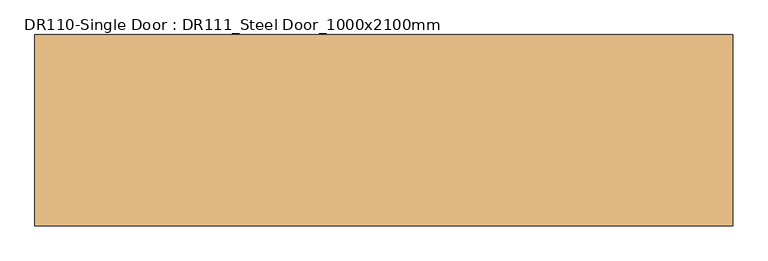
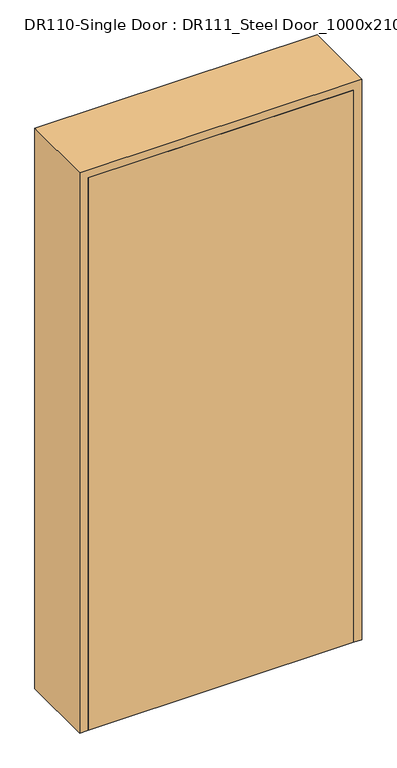
"""IFC4 building model written with IfcOpenShell, lengths in millimetres: door geometry, DR110-Single Door : DR111_Steel Door_1000x2100mm."""

from ifc_helpers import new_model, si_unit, origin, origin_with_axes, place, context, project, spatial, polyline, outline, extrude, faceted_brep, source, transform, mapped, element, save


def dr110_single_door_dr111_steel_door_1000x2100mm_c730d40a(model_context):
    return source(origin(), model_context, "Body", "SolidModel", [
        extrude(outline(polyline([(470.0, -137.0), (-470.0, -137.0), (-470.0, -102.0), (470.0, -102.0), (470.0, -137.0)])), origin_with_axes(), (0.0, 0.0, 1.0), 2070.0),
        faceted_brep([(470.0, -137.0, 0.0), (470.0, -102.0, 0.0), (450.0, -102.0, 0.0), (450.0, 102.0, 0.0), (470.0, 102.0, 0.0), (470.0, 137.0, 0.0), (500.0, 137.0, 0.0), (500.0, -137.0, 0.0), (500.0, -137.0, 2100.0), (-500.0, -137.0, 2100.0), (-500.0, -137.0, 0.0), (-470.0, -137.0, 0.0), (-470.0, -137.0, 2070.0), (470.0, -137.0, 2070.0), (500.0, 137.0, 2100.0), (470.0, 137.0, 2070.0), (-470.0, 137.0, 2070.0), (-470.0, 137.0, 0.0), (-500.0, 137.0, 0.0), (-500.0, 137.0, 2100.0), (470.0, 102.0, 2070.0), (450.0, 102.0, 2050.0), (-450.0, 102.0, 2050.0), (-450.0, 102.0, 0.0), (-470.0, 102.0, 0.0), (-470.0, 102.0, 2070.0), (450.0, -102.0, 2050.0), (470.0, -102.0, 2070.0), (-470.0, -102.0, 2070.0), (-470.0, -102.0, 0.0), (-450.0, -102.0, 0.0), (-450.0, -102.0, 2050.0)], [[[0, 1, 2, 3, 4, 5, 6, 7]], [[7, 8, 9, 10, 11, 12, 13, 0]], [[6, 14, 8, 7]], [[5, 15, 16, 17, 18, 19, 14, 6]], [[4, 20, 15, 5]], [[3, 21, 22, 23, 24, 25, 20, 4]], [[2, 26, 21, 3]], [[1, 27, 28, 29, 30, 31, 26, 2]], [[0, 13, 27, 1]], [[12, 11, 29, 28]], [[11, 10, 18, 17, 24, 23, 30, 29]], [[19, 18, 10, 9]], [[25, 24, 17, 16]], [[31, 30, 23, 22]], [[14, 19, 9, 8]], [[20, 25, 16, 15]], [[26, 31, 22, 21]], [[13, 12, 28, 27]]]),
    ])


if __name__ == "__main__":
    model = new_model("IFC4")
    model_context = context("Model", 3, world=origin())
    ifc_project = project(units=[si_unit("LENGTHUNIT", "METRE", prefix="MILLI")], contexts=[model_context])
    site = spatial("IfcSite", under=ifc_project)
    building = spatial("IfcBuilding", under=site)
    placement = place(None, origin())
    dr110_single_door_dr111_steel_door_1000x2100mm_shape = dr110_single_door_dr111_steel_door_1000x2100mm_c730d40a(model_context)
    element("IfcDoor", 1, ObjectType="DR110-Single Door : DR111_Steel Door_1000x2100mm", at=placement, inside=building, context=model_context, shape_type="MappedRepresentation", body=[
        mapped(dr110_single_door_dr111_steel_door_1000x2100mm_shape, transform((0.0, 0.0, 0.0), x_axis=(1.0, 0.0, 0.0), y_axis=(0.0, 1.0, 0.0), z_axis=(0.0, 0.0, 1.0))),
    ])
    save(model, "model.ifc")

# Revit data of these elements
# Type "DR110-Single Door : DR111_Steel Door_1000x2100mm"
#   Type Mark = "SD"
#   Analytic Construction = "<None>"
#   프레임 투영 외부. = 25 mm
#   프레임 투영 내부. = 25 mm
#   프레임 폭 = 75 mm
#   Height = 2100 mm
#   Width = 1000 mm
#   Define Thermal Properties by = 1
#   문 패널 = SD1 문 패널
#   문 프레임 = A04AQ098-00002_Steel Door_non FP_single
#   Function = (empty or 0)
#   Wall Closure = (empty or 0)
# Element 1 (IfcDoor, "DR110-Single Door : DR111_Steel Door_1000x2100mm")
#   Materials on its faces: "A04AQ098-00002_Steel Door_non FP_single", "SD1 문 패널"
# Materials
#   "SD1 문 패널": class "금속", colour RGB 247 247 247, transparency 0, Description = "STEEL DOOR (1000Wx2100H)"
#   "A04AQ098-00002_Steel Door_non FP_single": class "금속", colour RGB 247 247 247, transparency 0, Description = "Steel Door", W00) Work Master Code = "A04AQ098-00002", W01) Work Master_Lv1 = "Finishing Work", W02) Work Master_Lv2 = "Door & Window Work", W03) Work Master_Spec.1 = "Steel Door w/ Steel Frame", W04) Work Master_Spec.2 = "Fire Protective Rating: N/A, Single Door", W05) Work Master_Spec.3 = "w/ Hardware & Accessories", Cost = 0
